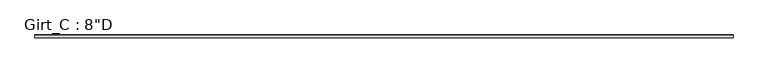
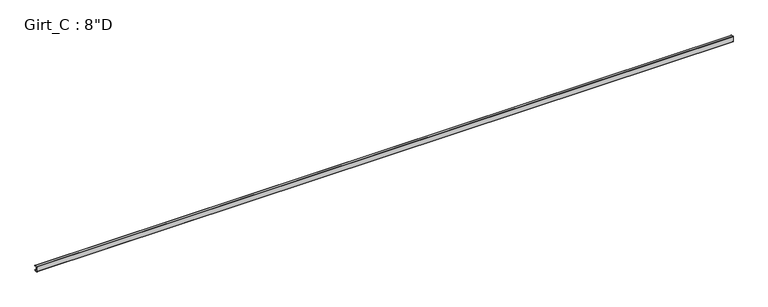
"""IFC4 building model written with IfcOpenShell, lengths in millimetres: beam geometry."""

from ifc_helpers import new_model, si_unit, point, frame, frame_2d, origin, place, context, project, spatial, polyline, circle_curve, trimmed, segment, composite_curve, outline, extrude, source, transform, mapped, element, save


def beam_d14e1dd8(model_context):
    return source(origin(), model_context, "Body", "SweptSolid", [
        extrude(outline(composite_curve([segment(polyline([(87.5109375, 101.6), (99.7560415, 87.0068534), (97.6278742, 85.221109), (86.2154765, 98.821875), (3.3005807, 98.821875)]), True, "CONTINUOUS"), segment(trimmed(circle_curve(frame_2d((3.3741066, 96.8381931)), 1.9850441), [point((3.3005807, 98.821875))], [point((1.3890625, 96.8381931))], True, "CARTESIAN"), True, "CONTINUOUS"), segment(polyline([(1.3890625, 96.8381931), (1.3890625, -96.8389339)]), True, "CONTINUOUS"), segment(trimmed(circle_curve(frame_2d((3.3748024, -96.8389339)), 1.9857399), [point((1.3890625, -96.8389339))], [point((3.2694106, -98.821875))], True, "CARTESIAN"), True, "CONTINUOUS"), segment(polyline([(3.2694106, -98.821875), (86.2154765, -98.821875), (97.6510975, -85.1934327), (99.7792647, -86.979177), (87.5109375, -101.6), (3.3734375, -101.6)]), True, "CONTINUOUS"), segment(trimmed(circle_curve(frame_2d((3.3734375, -96.8375)), 4.7625), [point((3.3734375, -101.6))], [point((-1.3890625, -96.8375))], False, "CARTESIAN"), True, "CONTINUOUS"), segment(polyline([(-1.3890625, -96.8375), (-1.3890625, 96.8375)]), True, "CONTINUOUS"), segment(trimmed(circle_curve(frame_2d((3.3734375, 96.8375)), 4.7625), [point((-1.3890625, 96.8375))], [point((3.3734375, 101.6))], False, "CARTESIAN"), True, "CONTINUOUS"), segment(polyline([(3.3734375, 101.6), (87.5109375, 101.6)]), True, "CONTINUOUS")], self_intersect=False)), frame((-12752.3875, 0.0, 0.0), z_axis=(1.0, 0.0, 0.0), x_axis=(0.0, 1.0, 0.0)), (0.0, 0.0, 1.0), 25403.175),
    ])


if __name__ == "__main__":
    model = new_model("IFC4")
    model_context = context("Model", 3, world=origin())
    ifc_project = project(units=[si_unit("LENGTHUNIT", "METRE", prefix="MILLI")], contexts=[model_context])
    site = spatial("IfcSite", under=ifc_project)
    building = spatial("IfcBuilding", under=site)
    placement = place(None, origin())
    beam_shape = beam_d14e1dd8(model_context)
    element("IfcBeam", 1, ObjectType="Girt_C : 8\"D", at=placement, inside=building, context=model_context, shape_type="MappedRepresentation", body=[
        mapped(beam_shape, transform((0.0, 0.0, 0.0), x_axis=(1.0, 0.0, 0.0), y_axis=(0.0, 1.0, 0.0), z_axis=(0.0, 0.0, 1.0))),
    ])
    save(model, "model.ifc")

# Revit data of these elements
# Type "Girt_C : 8\"D"
#   half leg = 0' - 1 3/4"
#   Web_Thickness = 0' - 0 7/64"
#   Length [instance default] = 10' - 0"
#   Leg_1 = 0' - 3 1/2"
#   Height = 0' - 8"
#   Structural Material [instance default] = none
# Element 1 (IfcBeam, "Girt_C : 8\"D")
#   Structural Material = CEE' SECTION (8.0x3.5C - SEE STRUCT. DWGS)
#   Materials on its faces: "CEE' SECTION (8.0x3.5C - SEE STRUCT. DWGS)"
# Materials
#   "CEE' SECTION (8.0x3.5C - SEE STRUCT. DWGS)": class "Metal", colour RGB 137 146 153, transparency 0, Description = "Steel, mill finish", Cost = 0
